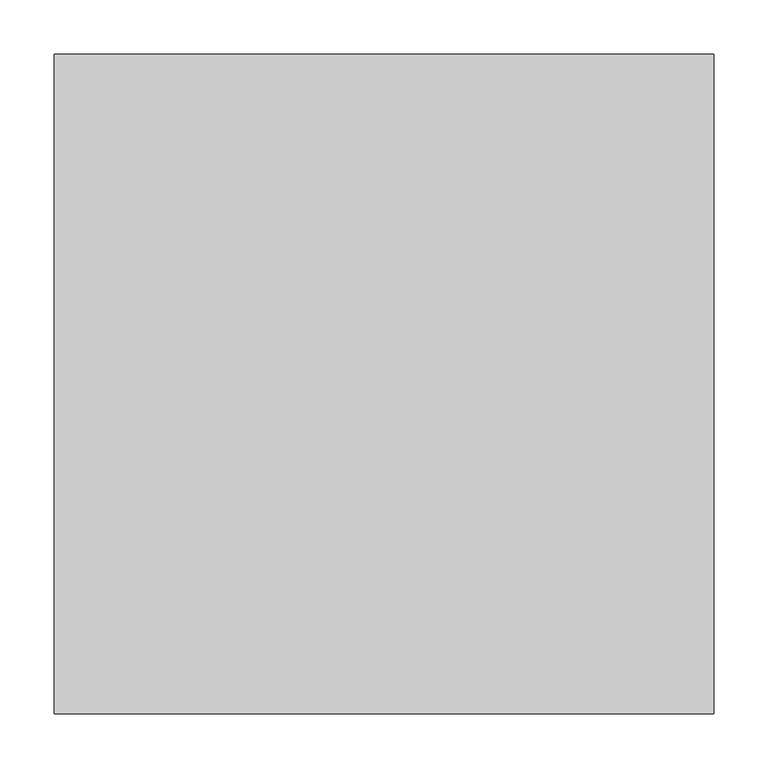
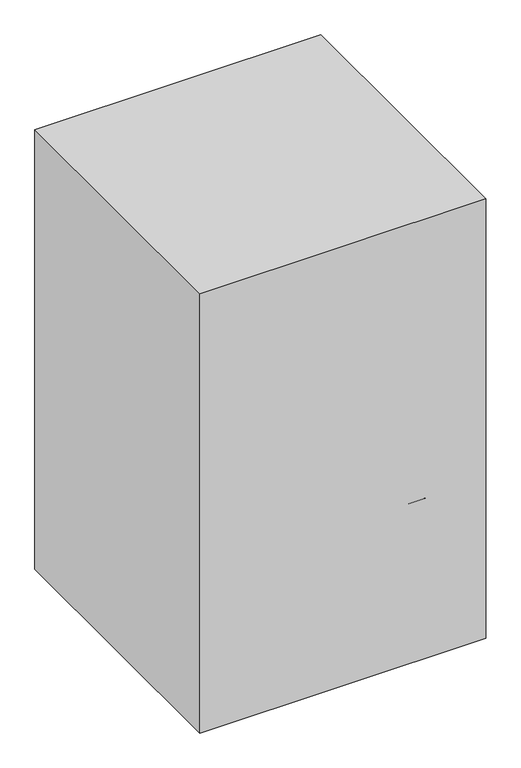
"""IFC4 building model written with IfcOpenShell, lengths in millimetres: proxy geometry, D3295 - Chair, Rotary, Laboratory, Dental : D3295 - Chair, Rotary, Laboratory, Dental."""

import ifcopenshell
import ifcopenshell.guid

model = None  # the IFC model being written
_history = None  # IfcOwnerHistory: only IFC2X3 demands one
_inside = {}  # id of a spatial element -> (the spatial element, [elements in it])
_under = {}  # id of a project, library or spatial element -> (it, [spatial elements below it])
_declared = {}  # id of a project -> (the project, [libraries it declares])
_typed = {}  # id of a type object -> (the type object, [elements of that type])
_made_of = {}  # id of a material, layer set ... -> (it, [elements and type objects made of it])


def new_model(schema):
    """Start an empty IFC model of exactly this schema.

    Asked for "IFC4X3", IfcOpenShell would pick the latest addendum, in which some entities
    have other attributes; the version numbers below select the first issue.
    IFC2X3 requires an IfcOwnerHistory on every rooted entity: one is made here for all.
    """
    global model, _history
    if schema == "IFC4X3":
        model = ifcopenshell.file(schema_version=(4, 3, 0, 0))
    else:
        model = ifcopenshell.file(schema=schema)
    _inside.clear()
    _under.clear()
    _declared.clear()
    _typed.clear()
    _made_of.clear()
    _history = None
    if model.schema == "IFC2X3":
        org = make("IfcOrganization", Name="unknown")
        user = make(
            "IfcPersonAndOrganization",
            ThePerson=make("IfcPerson", FamilyName="unknown"),
            TheOrganization=org,
        )
        app = make(
            "IfcApplication",
            ApplicationDeveloper=org,
            Version="unknown",
            ApplicationFullName="unknown",
            ApplicationIdentifier="unknown",
        )
        _history = make(
            "IfcOwnerHistory",
            OwningUser=user,
            OwningApplication=app,
            ChangeAction="ADDED",
            CreationDate=0,
        )
    return model


def make(cls, **values):
    """One entity of the class cls with the attributes given. An attribute that is None is left unset."""
    return model.create_entity(
        cls, **{name: value for name, value in values.items() if value is not None}
    )


def rooted(cls, **values):
    """An entity with a GlobalId (a new one), such as an element, a storey or a relation."""
    return make(cls, GlobalId=ifcopenshell.guid.new(), OwnerHistory=_history, **values)


def si_unit(unit_type, name, prefix=None):
    """IfcSIUnit, for example si_unit("LENGTHUNIT", "METRE", prefix="MILLI")."""
    return make("IfcSIUnit", UnitType=unit_type, Prefix=prefix, Name=name)


def assignment(units):
    """IfcUnitAssignment: the units of a project."""
    return None if units is None else make("IfcUnitAssignment", Units=units)


def point(xyz):
    """IfcCartesianPoint."""
    return None if xyz is None else make("IfcCartesianPoint", Coordinates=xyz)


def direction(xyz):
    """IfcDirection."""
    return None if xyz is None else make("IfcDirection", DirectionRatios=xyz)


def frame(location, z_axis=None, x_axis=None):
    """IfcAxis2Placement3D, a coordinate frame: its origin and axes. An axis left out is left unset."""
    return make(
        "IfcAxis2Placement3D",
        Location=point(location),
        Axis=direction(z_axis),
        RefDirection=direction(x_axis),
    )


def frame_2d(location, x_axis=None):
    """IfcAxis2Placement2D, a coordinate frame in the plane: its origin and x axis."""
    return make(
        "IfcAxis2Placement2D", Location=point(location), RefDirection=direction(x_axis)
    )


def origin():
    """The frame at (0, 0, 0) with its axes left unset."""
    return frame((0.0, 0.0, 0.0))


def origin_with_axes():
    """The frame at (0, 0, 0) with the z axis (0, 0, 1) and the x axis (1, 0, 0) written out."""
    return frame((0.0, 0.0, 0.0), z_axis=(0.0, 0.0, 1.0), x_axis=(1.0, 0.0, 0.0))


def place(relative_to, where):
    """IfcLocalPlacement: puts the frame where relative to a parent placement (None: the world)."""
    return make(
        "IfcLocalPlacement", PlacementRelTo=relative_to, RelativePlacement=where
    )


def context(
    kind, dimensions, precision=None, world=None, true_north=None, identifier=None
):
    """IfcGeometricRepresentationContext, for example the 3D "Model" context."""
    return make(
        "IfcGeometricRepresentationContext",
        ContextIdentifier=identifier,
        ContextType=kind,
        CoordinateSpaceDimension=dimensions,
        Precision=precision,
        WorldCoordinateSystem=world,
        TrueNorth=true_north,
    )


def project(units=None, contexts=None):
    """IfcProject with its units and contexts."""
    return rooted(
        "IfcProject",
        Name="project",
        RepresentationContexts=contexts,
        UnitsInContext=assignment(units),
    )


def spatial(cls, under=None, at=None, **own):
    """A site, building, storey or space (cls), placed at a placement, below another one or the project."""
    s = rooted(cls, ObjectPlacement=at, **own)
    if under is not None:
        _under.setdefault(under.id(), (under, []))[1].append(s)
    return s


def polyline(points):
    """IfcPolyline through the points."""
    return make("IfcPolyline", Points=[point(p) for p in points])


def circle_curve(where, radius):
    """IfcCircle in the frame where."""
    return make("IfcCircle", Position=where, Radius=radius)


def ellipse_curve(where, semi_axis1, semi_axis2):
    """IfcEllipse in the frame where."""
    return make(
        "IfcEllipse", Position=where, SemiAxis1=semi_axis1, SemiAxis2=semi_axis2
    )


def trimmed(basis, trim1, trim2, sense, master):
    """IfcTrimmedCurve: the piece of a basis curve between two trims."""
    return make(
        "IfcTrimmedCurve",
        BasisCurve=basis,
        Trim1=trim1,
        Trim2=trim2,
        SenseAgreement=sense,
        MasterRepresentation=master,
    )


def segment(curve, same_sense, transition):
    """IfcCompositeCurveSegment."""
    return make(
        "IfcCompositeCurveSegment",
        Transition=transition,
        SameSense=same_sense,
        ParentCurve=curve,
    )


def composite_curve(segments, self_intersect=None):
    """IfcCompositeCurve: segments joined end to end."""
    return make("IfcCompositeCurve", Segments=segments, SelfIntersect=self_intersect)


def outline(outer, holes=None, kind="AREA"):
    """IfcArbitraryClosedProfileDef: a profile drawn as a closed curve; with holes, ...WithVoids."""
    if holes is None:
        return make("IfcArbitraryClosedProfileDef", ProfileType=kind, OuterCurve=outer)
    return make(
        "IfcArbitraryProfileDefWithVoids",
        ProfileType=kind,
        OuterCurve=outer,
        InnerCurves=holes,
    )


def extrude(swept, where, along, depth):
    """IfcExtrudedAreaSolid: the profile swept, set in the frame where, extruded along a direction by depth."""
    return make(
        "IfcExtrudedAreaSolid",
        SweptArea=swept,
        Position=where,
        ExtrudedDirection=direction(along),
        Depth=depth,
    )


def shape(context_of_items, identifier, shape_type, items):
    """IfcShapeRepresentation: the items that make up one representation, for example the "Body"."""
    return make(
        "IfcShapeRepresentation",
        ContextOfItems=context_of_items,
        RepresentationIdentifier=identifier,
        RepresentationType=shape_type,
        Items=items,
    )


def source(mapping_origin, context_of_items, identifier, shape_type, items):
    """IfcRepresentationMap: a shape defined once, which mapped items show again and again."""
    return make(
        "IfcRepresentationMap",
        MappingOrigin=mapping_origin,
        MappedRepresentation=shape(context_of_items, identifier, shape_type, items),
    )


def transform(
    local_origin,
    x_axis=None,
    y_axis=None,
    z_axis=None,
    scale=None,
    scale2=None,
    scale3=None,
    uniform=True,
):
    """IfcCartesianTransformationOperator3D, or its non-uniform kind. x_axis, y_axis, z_axis: its Axis1, 2, 3."""
    if uniform:
        return make(
            "IfcCartesianTransformationOperator3D",
            Axis1=direction(x_axis),
            Axis2=direction(y_axis),
            LocalOrigin=point(local_origin),
            Scale=scale,
            Axis3=direction(z_axis),
        )
    return make(
        "IfcCartesianTransformationOperator3DnonUniform",
        Axis1=direction(x_axis),
        Axis2=direction(y_axis),
        LocalOrigin=point(local_origin),
        Scale=scale,
        Axis3=direction(z_axis),
        Scale2=scale2,
        Scale3=scale3,
    )


def mapped(mapping_source, mapping_target):
    """IfcMappedItem: shows the shape of a source again, moved by a transform."""
    return make(
        "IfcMappedItem", MappingSource=mapping_source, MappingTarget=mapping_target
    )


def made_of(thing, what):
    """Note that an element or type object is made of a material, layer set ...; save() writes the relation."""
    if what is not None:
        _made_of.setdefault(what.id(), (what, []))[1].append(thing)
    return thing


def element(
    cls,
    number,
    at=None,
    inside=None,
    cuts=None,
    type_object=None,
    material=None,
    context=None,
    identifier="Body",
    shape_type=None,
    held_by="IfcProductDefinitionShape",
    body=None,
    shapes=None,
    **own,
):
    """One element of the class cls, such as IfcWall. Its Tag is "e" and its number.

    at: its placement. inside: the storey or other place that contains it. cuts: it is an
    opening in that element (IfcRelVoidsElement). A single representation is given by context,
    identifier, shape_type and body (its items); several are given by shapes. held_by: the class
    of the entity that holds the representations. save() writes the other relations.
    """
    e = rooted(cls, Tag="e%d" % number, ObjectPlacement=at, **own)
    if body is not None:
        shapes = [shape(context, identifier, shape_type, body)]
    if shapes is not None:
        e.Representation = make(held_by, Representations=shapes)
    if inside is not None:
        _inside.setdefault(inside.id(), (inside, []))[1].append(e)
    if cuts is not None:
        rooted(
            "IfcRelVoidsElement", RelatingBuildingElement=cuts, RelatedOpeningElement=e
        )
    if type_object is not None:
        _typed.setdefault(type_object.id(), (type_object, []))[1].append(e)
    return made_of(e, material)


def aggregate(whole, parts):
    """IfcRelAggregates: a whole, such as a stair, and the parts it consists of."""
    return rooted("IfcRelAggregates", RelatingObject=whole, RelatedObjects=parts)


def save(model, path):
    """Write the relations noted so far, then the file.

    IfcRelAggregates (storeys below a building ...), IfcRelContainedInSpatialStructure (elements
    in a storey), IfcRelDefinesByType, IfcRelAssociatesMaterial and IfcRelDeclares: one each for
    every whole, place, type object, material and project.
    """
    for whole, parts in _under.values():
        aggregate(whole, parts)
    for where, things in _inside.values():
        rooted(
            "IfcRelContainedInSpatialStructure",
            RelatedElements=things,
            RelatingStructure=where,
        )
    for kind, things in _typed.values():
        rooted("IfcRelDefinesByType", RelatedObjects=things, RelatingType=kind)
    for what, things in _made_of.values():
        rooted("IfcRelAssociatesMaterial", RelatedObjects=things, RelatingMaterial=what)
    for by, libraries in _declared.values():
        rooted("IfcRelDeclares", RelatingContext=by, RelatedDefinitions=libraries)
    model.write(path)


def plane_surface(at):
    """IfcPlane: the flat surface through the origin of the frame at, square to its z axis."""
    return make("IfcPlane", Position=at)


def cylinder_surface(at, radius):
    """IfcCylindricalSurface: all points at the distance radius from the z axis of the frame at."""
    return make("IfcCylindricalSurface", Position=at, Radius=radius)


def revolved_surface(curve, axis_point, axis_direction):
    """IfcSurfaceOfRevolution: the curve turned about the line through axis_point along axis_direction."""
    return make(
        "IfcSurfaceOfRevolution",
        SweptCurve=make("IfcArbitraryOpenProfileDef", ProfileType="CURVE", Curve=curve),
        AxisPosition=make("IfcAxis1Placement", Location=point(axis_point), Axis=direction(axis_direction)),
    )


def advanced_brep(points, edges, surfaces, faces):
    """IfcAdvancedBrep: a solid bounded by faces that lie on surfaces and meet in shared edges.

    An edge is (start, end): straight between two places in points (the first is 0);
    or (start, end, curve); or (start, end, curve, False) where it runs against its curve.
    A face is (place in surfaces, loops), or (place, loops, False) where it looks against
    its surface's normal. A loop lists edges by number (the first is 1), with a minus sign
    where the edge is run from its end to its start. The first loop is the outer one.
    """
    corners = [point(p) for p in points]
    vertices = [make("IfcVertexPoint", VertexGeometry=c) for c in corners]
    made = []
    for start, end, *more in edges:
        made.append(
            make(
                "IfcEdgeCurve",
                EdgeStart=vertices[start],
                EdgeEnd=vertices[end],
                EdgeGeometry=more[0] if more else make("IfcPolyline", Points=[corners[start], corners[end]]),
                SameSense=more[1] if len(more) > 1 else True,
            )
        )
    hull = []
    for where, loops, *sense in faces:
        bounds = []
        for j, loop in enumerate(loops):
            ring = [make("IfcOrientedEdge", EdgeElement=made[abs(k) - 1], Orientation=k > 0) for k in loop]
            bounds.append(
                make(
                    "IfcFaceOuterBound" if j == 0 else "IfcFaceBound",
                    Bound=make("IfcEdgeLoop", EdgeList=ring),
                    Orientation=True,
                )
            )
        hull.append(make("IfcAdvancedFace", Bounds=bounds, FaceSurface=surfaces[where], SameSense=sense[0] if sense else True))
    return make("IfcAdvancedBrep", Outer=make("IfcClosedShell", CfsFaces=hull))


def specialty_equipment_0317cfd4(model_context):
    return source(origin(), model_context, "Body", "SolidModel", [
        advanced_brep(
        [(20.5891067, -39.0088165, 158.3164474), (20.5891067, -39.0088165, 212.7487443), (12.606954, -21.8910347, 212.7487443), (12.606954, -21.8910347, 158.3164474), (283.7284885, 83.6950923, 57.6571213), (283.7284885, 83.6950923, 86.0096871), (287.501904, 95.8556376, 82.2734822), (275.3053581, 100.6072429, 86.2220806), (275.3053581, 100.6072429, 57.8258095), (287.501904, 95.8556376, 54.689734)],
        [
            (0, 1),
            (1, 2),
            (2, 3),
            (3, 0),
            (0, 4),
            (4, 5),
            (5, 1),
            (5, 6, ellipse_curve(frame((278.918781, 91.8532617, 86.4074773), z_axis=(0.3625792018206629, 0.16907345849670724, 0.9164881276039822), x_axis=(0.8306203267741233, 0.3873246193939933, -0.40006188516396646)), 10.333389, 9.4704283)),
            (6, 7, ellipse_curve(frame((278.918781, 91.8532617, 86.4074773), z_axis=(0.3625792018206629, 0.16907345849670724, 0.9164881276039822), x_axis=(0.8306203267741233, 0.3873246193939933, -0.40006188516396646)), 10.333389, 9.4704283)),
            (7, 2),
            (7, 8),
            (8, 3),
            (8, 9, ellipse_curve(frame((278.918781, 91.8532617, 57.9730562), z_axis=(-0.2968743688836678, -0.13843479172039067, -0.9448287768380342), x_axis=(0.8563056778646188, 0.3993018953098915, -0.3275646233321667)), 10.0234334, 9.4704283)),
            (9, 4, ellipse_curve(frame((278.918781, 91.8532617, 57.9730562), z_axis=(-0.2968743688836678, -0.13843479172039067, -0.9448287768380342), x_axis=(0.8563056778646188, 0.3993018953098915, -0.3275646233321667)), 10.0234334, 9.4704283)),
            (6, 9),
        ],
        [
            plane_surface(frame((16.5980304, -30.4499256, 185.5325958), z_axis=(-0.9063077870366449, -0.42261826174071043, 0.0), x_axis=(-0.42261826174071043, 0.9063077870366449, 0.0))),
            plane_surface(frame((20.5891067, -39.0088165, 185.5325958), z_axis=(0.4226182617407104, -0.9063077870366448, 0.0), x_axis=(0.0, 0.0, 1.0))),
            plane_surface(frame((16.5980304, -30.4499256, 212.7487443), z_axis=(0.36257920182066294, 0.16907345849670727, 0.9164881276039825), x_axis=(-0.42261826174071043, 0.9063077870366449, 0.0))),
            plane_surface(frame((12.606954, -21.8910347, 185.5325958), z_axis=(-0.4226182617407102, 0.906307787036645, 0.0), x_axis=(0.0, 0.0, -1.0))),
            plane_surface(frame((16.5980304, -30.4499256, 158.3164474), z_axis=(-0.29687436888366786, -0.1384347917203907, -0.9448287768380345), x_axis=(0.42261826174071043, -0.9063077870366449, 0.0))),
            cylinder_surface(frame((278.918781, 91.8532617, 0.0), z_axis=(0.0, 0.0, -1.0000000000000002), x_axis=(-0.9063077870366449, -0.42261826174071043, 0.0)), 9.4704283),
        ],
        [
            (0, [[1, 2, 3, 4]]),
            (1, [[5, 6, 7, -1]]),
            (2, [[-7, 8, 9, 10, -2]]),
            (3, [[-10, 11, 12, -3]]),
            (4, [[-12, 13, 14, -5, -4]]),
            (5, [[-13, -11, -9, 15]]),
            (5, [[-8, -6, -14, -15]]),
        ],
    ),
        extrude(outline(composite_curve([segment(trimmed(circle_curve(frame_2d((-0.4565328, -38.3009494)), 25.4), [point((24.9434672, -38.3009494))], [point((-25.8565328, -38.3009494))], False, "CARTESIAN"), True, "CONTINUOUS"), segment(trimmed(circle_curve(frame_2d((-0.4565328, -38.3009494)), 25.4), [point((-25.8565328, -38.3009494))], [point((24.9434672, -38.3009494))], False, "CARTESIAN"), True, "CONTINUOUS")], self_intersect=False)), frame((0.0, 0.0, 154.0271692), z_axis=(0.0, 0.0, 1.0), x_axis=(1.0, 0.0, 0.0)), (0.0, 0.0, 1.0), 58.7215752),
        advanced_brep(
        [(-229.5082147, 153.1947504, 328.6387079), (-229.5082147, 178.826585, 331.293346), (236.3508412, 177.6557493, 331.1720849), (232.0214447, 152.7605661, 328.5937403), (-229.5082147, 246.1177228, 855.6310718), (232.0214447, 245.7251028, 855.8218273), (236.3508412, 268.237077, 844.8843217), (-229.5082147, 269.2958289, 844.3699241)],
        [
            (0, 1, circle_curve(frame((-229.5082147, 166.0106677, 329.9660269), z_axis=(0.0, 0.10301698777210262, -0.9946795967699159), x_axis=(-1.0, 0.0, 0.0)), 12.8844679)),
            (1, 2, circle_curve(frame((0.0, -1168.6045098, 191.7425871), z_axis=(0.0, 0.10301698777210262, -0.9946795967699159), x_axis=(-1.0, 0.0, 0.0)), 1373.9428628)),
            (2, 3, circle_curve(frame((232.0214447, 165.5806144, 329.9214872), z_axis=(0.0, 0.10301698777210262, -0.9946795967699159), x_axis=(-1.0, 0.0, 0.0)), 12.888621)),
            (3, 0, circle_curve(frame((0.0, -1168.6045098, 191.7425871), z_axis=(0.0, -0.10301698777210262, 0.9946795967699159), x_axis=(-1.0, 0.0, 0.0)), 1348.5428628)),
            (4, 5, circle_curve(frame((0.0, -949.1460573, 1436.3533187), z_axis=(0.0, -0.4370047614753844, -0.8994591922082082), x_axis=(-1.0, 0.0, 0.0)), 1348.5428628)),
            (5, 6, circle_curve(frame((232.0214447, 257.3178914, 850.1894385), z_axis=(0.0, 0.4370047614753844, 0.8994591922082082), x_axis=(-1.0, 0.0, 0.0)), 12.888621)),
            (6, 7, circle_curve(frame((0.0, -949.1460573, 1436.3533187), z_axis=(0.0, 0.4370047614753844, 0.8994591922082082), x_axis=(-1.0, 0.0, 0.0)), 1373.9428628)),
            (7, 4, circle_curve(frame((-229.5082147, 257.7067759, 850.0004979), z_axis=(0.0, 0.4370047614753844, 0.8994591922082082), x_axis=(-1.0, 0.0, 0.0)), 12.8844679)),
            (4, 0, circle_curve(frame((-229.5082147, 1123.8751957, 429.1701512), z_axis=(1.0, 0.0, 0.0), x_axis=(0.0, -0.9946795967699159, -0.10301698777210261)), 975.8724803)),
            (3, 5, circle_curve(frame((232.0214447, 1123.8751957, 429.1701512), z_axis=(-1.0, 0.0, 0.0), x_axis=(0.0, -0.9946795967699159, -0.10301698777210261)), 976.308987)),
            (2, 6, circle_curve(frame((236.3508412, 1123.8751957, 429.1701512), z_axis=(-1.0, 0.0, 0.0), x_axis=(0.0, -0.9946795967699159, -0.10301698777210261)), 951.280643)),
            (1, 7, circle_curve(frame((-229.5082147, 1123.8751957, 429.1701512), z_axis=(-1.0, 0.0, 0.0), x_axis=(0.0, -0.9946795967699159, -0.10301698777210261)), 950.1035446)),
        ],
        [
            plane_surface(frame((-317.5, 135.0564347, 326.7601586), z_axis=(0.0, 0.10301698777210258, -0.994679596769916), x_axis=(-1.0, 0.0, 0.0))),
            plane_surface(frame((-317.5, 229.715783, 863.6), z_axis=(0.0, 0.4370047614753844, 0.8994591922082082), x_axis=(-1.0, 0.0, 0.0))),
            revolved_surface(trimmed(ellipse_curve(frame((0.0, -1168.6045098, 191.7425871), z_axis=(0.0, 0.10301698777210262, -0.9946795967699159), x_axis=(-1.0, 0.0, 0.0)), 1348.5428628, 1348.5428628), [point((-229.5082147, 153.1947504, 328.6387079))], [point((232.0214447, 152.7605661, 328.5937403))], True, "CARTESIAN"), (-317.5, 1123.8751957, 429.1701512), (1.0, 0.0, 0.0)),
            revolved_surface(trimmed(ellipse_curve(frame((232.0214447, 165.5806144, 329.9214872), z_axis=(0.0, -0.10301698777210262, 0.9946795967699159), x_axis=(-1.0, 0.0, 0.0)), 12.888621, 12.888621), [point((232.0214447, 152.7605661, 328.5937403))], [point((236.3508412, 177.6557493, 331.1720849))], True, "CARTESIAN"), (-317.5, 1123.8751957, 429.1701512), (1.0, 0.0, 0.0)),
            revolved_surface(trimmed(ellipse_curve(frame((0.0, -1168.6045098, 191.7425871), z_axis=(0.0, -0.10301698777210262, 0.9946795967699159), x_axis=(-1.0, 0.0, 0.0)), 1373.9428628, 1373.9428628), [point((236.3508412, 177.6557493, 331.1720849))], [point((-229.5082147, 178.826585, 331.293346))], True, "CARTESIAN"), (-317.5, 1123.8751957, 429.1701512), (1.0, 0.0, 0.0)),
            revolved_surface(trimmed(ellipse_curve(frame((-229.5082147, 166.0106677, 329.9660269), z_axis=(0.0, -0.10301698777210262, 0.9946795967699159), x_axis=(-1.0, 0.0, 0.0)), 12.8844679, 12.8844679), [point((-229.5082147, 178.826585, 331.293346))], [point((-229.5082147, 153.1947504, 328.6387079))], True, "CARTESIAN"), (-317.5, 1123.8751957, 429.1701512), (1.0, 0.0, 0.0)),
        ],
        [
            (0, [[1, 2, 3, 4]]),
            (1, [[5, 6, 7, 8]]),
            (2, [[-5, 9, -4, 10]]),
            (3, [[-6, -10, -3, 11]]),
            (4, [[-7, -11, -2, 12]]),
            (5, [[-8, -12, -1, -9]]),
        ],
    ),
        extrude(outline(composite_curve([segment(polyline([(-213.079753, 135.9379297), (221.4112726, 135.9379297), (221.4112726, -221.0075832)]), True, "CONTINUOUS"), segment(trimmed(circle_curve(frame_2d((194.6657598, -221.0075832)), 26.7455128), [point((221.4112726, -221.0075832))], [point((194.6657598, -247.753096))], False, "CARTESIAN"), True, "CONTINUOUS"), segment(polyline([(194.6657598, -247.753096), (-186.3342402, -247.753096)]), True, "CONTINUOUS"), segment(trimmed(circle_curve(frame_2d((-186.3342402, -221.0075832)), 26.7455128), [point((-186.3342402, -247.753096))], [point((-213.079753, -221.0075832))], False, "CARTESIAN"), True, "CONTINUOUS"), segment(polyline([(-213.079753, -221.0075832), (-213.079753, 135.9379297)]), True, "CONTINUOUS")], self_intersect=False)), frame((0.0, 0.0, 324.0440254), z_axis=(0.0, 0.0, 1.0), x_axis=(1.0, 0.0, 0.0)), (0.0, 0.0, 1.0), 67.8491407),
        advanced_brep(
        [(-213.079753, 134.5924168, 391.8931661), (-213.079753, 134.5924168, 324.0440254), (-211.7342402, 135.9379297, 324.0440254), (-211.7342402, 135.9379297, 391.8931661), (-213.079753, -221.0075832, 391.8931661), (-213.079753, -221.0075832, 324.0440254), (-186.3342402, -247.753096, 391.8931661), (-186.3342402, -247.753096, 324.0440254), (194.6657598, -247.753096, 391.8931661), (194.6657598, -247.753096, 324.0440254), (221.4112726, -221.0075832, 391.8931661), (221.4112726, -221.0075832, 324.0440254), (221.4112726, 134.5924168, 391.8931661), (221.4112726, 134.5924168, 324.0440254), (220.0657598, 135.9379297, 391.8931661), (220.0657598, 135.9379297, 324.0440254)],
        [
            (0, 1),
            (1, 2, circle_curve(frame((-211.7342402, 134.5924168, 324.0440254), z_axis=(0.0, 0.0, -1.0), x_axis=(0.0, 1.0, 0.0)), 1.3455128)),
            (2, 3),
            (3, 0, circle_curve(frame((-211.7342402, 134.5924168, 391.8931661), z_axis=(0.0, 0.0, 1.0), x_axis=(0.0, 1.0, 0.0)), 1.3455128)),
            (1, 0, circle_curve(frame((-213.079753, 134.5924168, 357.9685958), z_axis=(0.0, 1.0, 0.0), x_axis=(1.0, 0.0, 0.0)), 33.9245703)),
            (3, 2, circle_curve(frame((-211.7342402, 135.9379297, 357.9685958), z_axis=(-1.0, 0.0, 0.0), x_axis=(0.0, -1.0, 0.0)), 33.9245703)),
            (0, 4),
            (4, 5),
            (5, 1),
            (5, 4, circle_curve(frame((-213.079753, -221.0075832, 357.9685958), z_axis=(0.0, 1.0, 0.0), x_axis=(1.0, 0.0, 0.0)), 33.9245703)),
            (6, 7),
            (7, 5, circle_curve(frame((-186.3342402, -221.0075832, 324.0440254), z_axis=(0.0, 0.0, -1.0), x_axis=(-1.0, 0.0, 0.0)), 26.7455128)),
            (4, 6, circle_curve(frame((-186.3342402, -221.0075832, 391.8931661), z_axis=(0.0, 0.0, 1.0), x_axis=(-1.0, 0.0, 0.0)), 26.7455128)),
            (7, 6, circle_curve(frame((-186.3342402, -247.753096, 357.9685958), z_axis=(-1.0, 0.0, 0.0), x_axis=(0.0, 1.0, 0.0)), 33.9245703)),
            (6, 8),
            (8, 9),
            (9, 7),
            (9, 8, circle_curve(frame((194.6657598, -247.753096, 357.9685958), z_axis=(-1.0, 0.0, 0.0), x_axis=(0.0, 1.0, 0.0)), 33.9245703)),
            (10, 11),
            (11, 9, circle_curve(frame((194.6657598, -221.0075832, 324.0440254), z_axis=(0.0, 0.0, -1.0), x_axis=(0.0, -1.0, 0.0)), 26.7455128)),
            (8, 10, circle_curve(frame((194.6657598, -221.0075832, 391.8931661), z_axis=(0.0, 0.0, 1.0), x_axis=(0.0, -1.0, 0.0)), 26.7455128)),
            (11, 10, circle_curve(frame((221.4112726, -221.0075832, 357.9685958), z_axis=(0.0, -1.0, 0.0), x_axis=(-1.0, 0.0, 0.0)), 33.9245703)),
            (10, 12),
            (12, 13),
            (13, 11),
            (13, 12, circle_curve(frame((221.4112726, 134.5924168, 357.9685958), z_axis=(0.0, -1.0, 0.0), x_axis=(-1.0, 0.0, 0.0)), 33.9245703)),
            (14, 15),
            (15, 13, circle_curve(frame((220.0657598, 134.5924168, 324.0440254), z_axis=(0.0, 0.0, -1.0), x_axis=(1.0, 0.0, 0.0)), 1.3455128)),
            (12, 14, circle_curve(frame((220.0657598, 134.5924168, 391.8931661), z_axis=(0.0, 0.0, 1.0), x_axis=(1.0, 0.0, 0.0)), 1.3455128)),
            (15, 14, circle_curve(frame((220.0657598, 135.9379297, 357.9685958), z_axis=(1.0, 0.0, 0.0), x_axis=(0.0, -1.0, 0.0)), 33.9245703)),
            (14, 3),
            (2, 15),
        ],
        [
            revolved_surface(polyline([(-211.7342402, 135.9379296, 324.0440254), (-211.7342402, 135.9379296, 391.8931661)]), (-211.7342402, 134.5924168, 0.0), (0.0, 0.0, -1.0)),
            revolved_surface(trimmed(ellipse_curve(frame((-211.7342402, 135.9379297, 357.9685958), z_axis=(-1.0, 0.0, 0.0), x_axis=(0.0, -1.0, 0.0)), 33.9245703, 33.9245703), [point((-211.7342402, 135.9379297, 391.8931661))], [point((-211.7342402, 135.9379297, 324.0440254))], True, "CARTESIAN"), (-211.7342402, 134.5924168, 0.0), (0.0, 0.0, -1.0)),
            plane_surface(frame((-213.079753, 134.5924168, 324.0440254), z_axis=(1.0, 0.0, 0.0), x_axis=(0.0, -1.0, 0.0))),
            cylinder_surface(frame((-213.079753, 134.5924168, 357.9685958), z_axis=(0.0, 1.0, 0.0), x_axis=(1.0, 0.0, 0.0)), 33.9245703),
            revolved_surface(polyline([(-213.079753, -221.0075832, 324.0440254), (-213.079753, -221.0075832, 391.8931661)]), (-186.3342402, -221.0075832, 0.0), (0.0, 0.0, -1.0)),
            revolved_surface(trimmed(ellipse_curve(frame((-213.079753, -221.0075832, 357.9685958), z_axis=(0.0, -1.0, 0.0), x_axis=(1.0, 0.0, 0.0)), 33.9245703, 33.9245703), [point((-213.079753, -221.0075832, 391.8931661))], [point((-213.079753, -221.0075832, 324.0440254))], True, "CARTESIAN"), (-186.3342402, -221.0075832, 0.0), (0.0, 0.0, -1.0)),
            plane_surface(frame((-186.3342402, -247.753096, 324.0440254), z_axis=(0.0, 1.0, 0.0), x_axis=(1.0, 0.0, 0.0))),
            cylinder_surface(frame((-186.3342402, -247.753096, 357.9685958), z_axis=(-1.0, 0.0, 0.0), x_axis=(0.0, 1.0, 0.0)), 33.9245703),
            revolved_surface(polyline([(194.6657598, -247.753096, 324.0440254), (194.6657598, -247.753096, 391.8931661)]), (194.6657598, -221.0075832, 0.0), (0.0, 0.0, -1.0)),
            revolved_surface(trimmed(ellipse_curve(frame((194.6657598, -247.753096, 357.9685958), z_axis=(1.0, 0.0, 0.0), x_axis=(0.0, 1.0, 0.0)), 33.9245703, 33.9245703), [point((194.6657598, -247.753096, 391.8931661))], [point((194.6657598, -247.753096, 324.0440254))], True, "CARTESIAN"), (194.6657598, -221.0075832, 0.0), (0.0, 0.0, -1.0)),
            plane_surface(frame((221.4112726, -221.0075832, 324.0440254), z_axis=(-1.0, 0.0, 0.0), x_axis=(0.0, 1.0, 0.0))),
            cylinder_surface(frame((221.4112726, -221.0075832, 357.9685958), z_axis=(0.0, -1.0, 0.0), x_axis=(-1.0, 0.0, 0.0)), 33.9245703),
            revolved_surface(polyline([(221.4112726, 134.5924168, 324.0440254), (221.4112726, 134.5924168, 391.8931661)]), (220.0657598, 134.5924168, 0.0), (0.0, 0.0, -1.0)),
            revolved_surface(trimmed(ellipse_curve(frame((221.4112726, 134.5924168, 357.9685958), z_axis=(0.0, 1.0, 0.0), x_axis=(-1.0, 0.0, 0.0)), 33.9245703, 33.9245703), [point((221.4112726, 134.5924168, 391.8931661))], [point((221.4112726, 134.5924168, 324.0440254))], True, "CARTESIAN"), (220.0657598, 134.5924168, 0.0), (0.0, 0.0, -1.0)),
            plane_surface(frame((220.0657598, 135.9379297, 324.0440254), z_axis=(0.0, -1.0, 0.0), x_axis=(-1.0, 0.0, 0.0))),
            cylinder_surface(frame((220.0657598, 135.9379297, 357.9685958), z_axis=(1.0, 0.0, 0.0), x_axis=(0.0, -1.0, 0.0)), 33.9245703),
        ],
        [
            (0, [[1, 2, 3, 4]]),
            (1, [[5, -4, 6, -2]]),
            (2, [[7, 8, 9, -1]]),
            (3, [[-9, 10, -7, -5]]),
            (4, [[11, 12, -8, 13]]),
            (5, [[14, -13, -10, -12]]),
            (6, [[15, 16, 17, -11]]),
            (7, [[-17, 18, -15, -14]]),
            (8, [[19, 20, -16, 21]]),
            (9, [[22, -21, -18, -20]]),
            (10, [[23, 24, 25, -19]]),
            (11, [[-25, 26, -23, -22]]),
            (12, [[27, 28, -24, 29]]),
            (13, [[30, -29, -26, -28]]),
            (14, [[31, -3, 32, -27]]),
            (15, [[-32, -6, -31, -30]]),
        ],
    ),
        extrude(outline(composite_curve([segment(trimmed(circle_curve(frame_2d((0.0, -38.1)), 12.7), [point((12.7, -38.1))], [point((-12.7, -38.1))], False, "CARTESIAN"), True, "CONTINUOUS"), segment(trimmed(circle_curve(frame_2d((0.0, -38.1)), 12.7), [point((-12.7, -38.1))], [point((12.7, -38.1))], False, "CARTESIAN"), True, "CONTINUOUS")], self_intersect=False)), frame((0.0, 0.0, 212.7487443), z_axis=(0.0, 0.0, 1.0), x_axis=(1.0, 0.0, 0.0)), (0.0, 0.0, 1.0), 66.217703),
        extrude(outline(polyline([(304.8, -304.8), (-304.8, -304.8), (-304.8, 304.8), (304.8, 304.8), (304.8, -304.8)])), origin_with_axes(), (0.0, 0.0, 1.0), 990.6),
    ])


if __name__ == "__main__":
    model = new_model("IFC4")
    model_context = context("Model", 3, world=origin())
    ifc_project = project(units=[si_unit("LENGTHUNIT", "METRE", prefix="MILLI")], contexts=[model_context])
    site = spatial("IfcSite", under=ifc_project)
    building = spatial("IfcBuilding", under=site)
    placement = place(None, origin())
    specialty_equipment_shape = specialty_equipment_0317cfd4(model_context)
    element("IfcBuildingElementProxy", 1, Name="D3295 - Chair, Rotary, Laboratory, Dental : D3295 - Chair, Rotary, Laboratory, Dental", ObjectType="D3295 - Chair, Rotary, Laboratory, Dental : D3295 - Chair, Rotary, Laboratory, Dental", at=placement, inside=building, context=model_context, shape_type="MappedRepresentation", body=[
        mapped(specialty_equipment_shape, transform((0.0, 0.0, 0.0), x_axis=(1.0, 0.0, 0.0), y_axis=(0.0, 1.0, 0.0), z_axis=(0.0, 0.0, 1.0))),
    ])
    save(model, "model.ifc")

# Revit data of these elements
# Project information
#   Sheets - Total = "6"
#   Project Issue Date = "Issue Date"
#   Project Status = "Project Status"
#   Client Name = "Owner"
#   Project Address = "Enter address here"
#   Project Name = "Project Name"
#   Project Number = "Project Number"
#   Publication Date = "30-Jan-15"
# Type "D3295 - Chair, Rotary, Laboratory, Dental : D3295 - Chair, Rotary, Laboratory, Dental"
#   Watts2 = "0"
#   Watts1 = "0"
#   Unit_Issue = "EA"
#   UTIL_6_Misc = "-"
#   UTIL_5_NonMedGas = "-"
#   UTIL_4_MiscGas = "-"
#   UTIL_3_MedGas = "-"
#   UTIL_2_Elec = "-"
#   UTIL_1_WaterDrain = "-"
#   Nomenclature = "Chair, Rotary, Laboratory, Dental"
#   NSN = "6520"
#   Location [instance default] = ""
#   JSN = "D3295"
#   Fund_Source_VA = "-"
#   Fund_Source_Navy = "-"
#   Fund_Source_Army = "-"
#   Fund_Source_AF = "-"
#   ELEC_Volts2 = "0"
#   ELEC_Volts1 = "0"
#   ELEC_Phase2 = "0"
#   ELEC_Phase1 = "0"
#   ELEC_HertzSwitch = "0"
#   ELEC_HertzDependent = "0"
#   ELEC_Hertz = "0"
#   ELEC_Amps2 = "0"
#   ELEC_Amps1 = "0"
#   DetailDescription = "Rotary dental laboratory chair. The chair is used by technicians while working at a bench. Chairs also have casters and an adjustable backrest."
#   CAT_VA = "C"
#   CAT_Navy = "C"
#   CAT_IHS = "-"
#   CAT_Army = "C"
#   CAT_AF = "C"
#   BTUperhour = "0"
#   Weight_IP = 36
#   DIM_Width_IP = 2' - 0"
#   DIM_Height_IP = 3' - 0"
#   DIM_Depth_IP = 2' - 0"
#   Assembly Code = ""
# Element 1 (IfcBuildingElementProxy, "D3295 - Chair, Rotary, Laboratory, Dental : D3295 - Chair, Rotary, Laboratory, Dental")
#   Location = "DNPL2"
#   Materials on its faces: "00 - bernhardt blitz - base", "00 - bernhardt blitz - Seat Fabric", "00 - bernhardt blitz - wheels", "00 - bernhardt blitz - arms", "00 - bernhardt blitz - mechanic", "00 - bernhardt blitz - Back Fabric", "EquipSpace"
# Materials
#   "00 - bernhardt blitz - base": class "Miscellaneous", colour RGB 192 192 192, transparency 0
#   "00 - bernhardt blitz - Seat Fabric": class "Miscellaneous", colour RGB 188 173 117, transparency 0
#   "00 - bernhardt blitz - wheels": class "Miscellaneous", colour RGB 51 51 51, transparency 0
#   "00 - bernhardt blitz - arms": class "Miscellaneous", colour RGB 51 51 51, transparency 0
#   "00 - bernhardt blitz - mechanic": class "Miscellaneous", colour RGB 62 62 62, transparency 0
#   "00 - bernhardt blitz - Back Fabric": class "Miscellaneous", colour RGB 93 93 93, transparency 0
#   "EquipSpace": class "Unassigned", colour RGB 221 217 195, transparency 0.5
